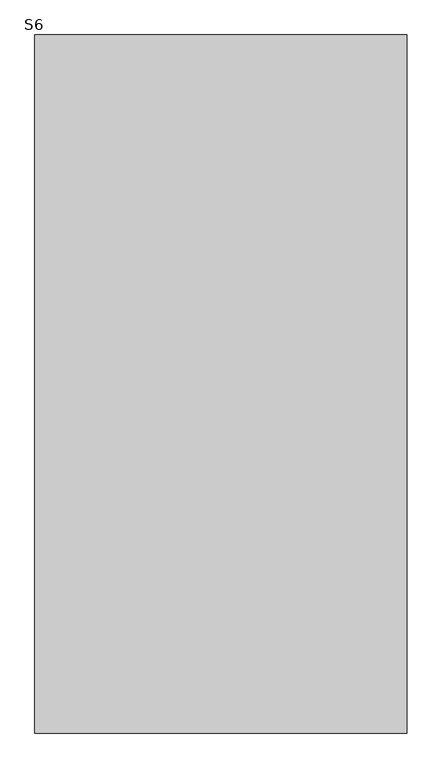
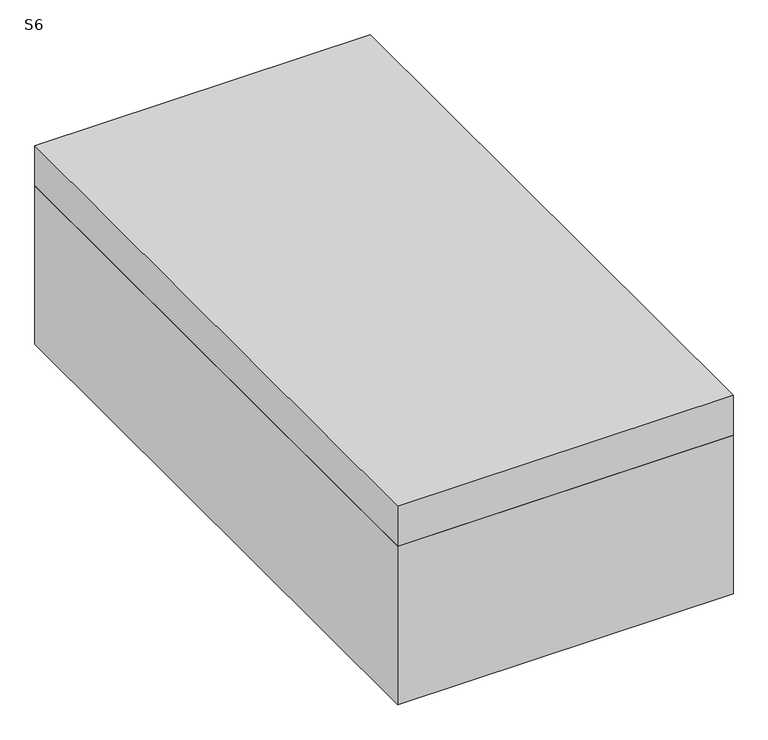
"""IFC4 building model written with IfcOpenShell, lengths in millimetres: fastener geometry, TQS - Sapata : S6."""

from ifc_helpers import new_model, si_unit, frame, origin, place, context, project, spatial, polyline, outline, extrude, source, transform, mapped, element, save


def s6_dd942dc6(model_context):
    return source(origin(), model_context, "Body", "SweptSolid", [
        extrude(outline(polyline([(200.0, 550.0), (200.0, -950.0), (-600.0, -950.0), (-600.0, 550.0), (200.0, 550.0)])), frame((0.0, 0.0, -100.0), z_axis=(0.0, 0.0, 1.0), x_axis=(1.0, 0.0, 0.0)), (0.0, 0.0, 1.0), 100.0),
        extrude(outline(polyline([(200.0, 550.0), (200.0, -950.0), (-600.0, -950.0), (-600.0, 550.0), (200.0, 550.0)])), frame((0.0, 0.0, -500.0), z_axis=(0.0, 0.0, 1.0), x_axis=(1.0, 0.0, 0.0)), (0.0, 0.0, 1.0), 400.0),
    ])


if __name__ == "__main__":
    model = new_model("IFC4")
    model_context = context("Model", 3, world=origin())
    ifc_project = project(units=[si_unit("LENGTHUNIT", "METRE", prefix="MILLI")], contexts=[model_context])
    site = spatial("IfcSite", under=ifc_project)
    building = spatial("IfcBuilding", under=site)
    placement = place(None, origin())
    s6_shape = s6_dd942dc6(model_context)
    element("IfcFastener", 1, ObjectType="TQS - Sapata : S6", at=placement, inside=building, context=model_context, shape_type="MappedRepresentation", body=[
        mapped(s6_shape, transform((0.0, 0.0, 0.0), x_axis=(1.0, 0.0, 0.0), y_axis=(0.0, 1.0, 0.0), z_axis=(0.0, 0.0, 1.0))),
    ])
    save(model, "model.ifc")

# Revit data of these elements
# Type "TQS - Sapata : S6"
#   TY = 1.50 m
#   TX = 0.80 m
#   HS = 0.50 m
#   H0 = 0.40 m
#   EXCYABS = 0.75 m
#   EXCY = 0.00 m
#   EXCXABS = 0.40 m
#   EXCX = 0.00 m
#   DIMY = 1.50 m
#   DIMX = 0.80 m
#   Material estrutural = Concreto - Concreto concretado no local
#   Width = 0
#   Length = 0
# Element 1 (IfcFastener, "TQS - Sapata : S6")
#   Materials on its faces: "Concreto - Concreto concretado no local"
# Materials
#   "Concreto - Concreto concretado no local": class "Concreto", colour RGB 192 192 192, transparency 0
